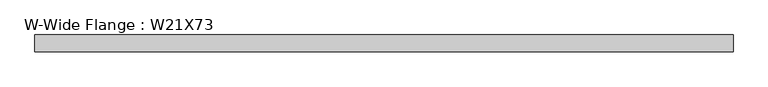
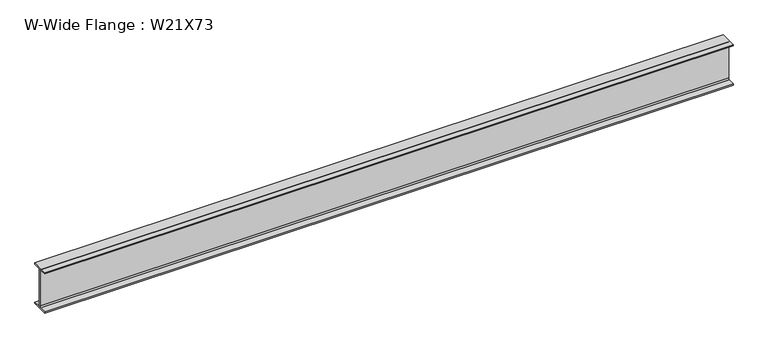
"""IFC4 building model written with IfcOpenShell, lengths in millimetres: beam geometry, W-Wide Flange : W21X73."""

import ifcopenshell
import ifcopenshell.guid

model = None  # the IFC model being written
_history = None  # IfcOwnerHistory: only IFC2X3 demands one
_inside = {}  # id of a spatial element -> (the spatial element, [elements in it])
_under = {}  # id of a project, library or spatial element -> (it, [spatial elements below it])
_declared = {}  # id of a project -> (the project, [libraries it declares])
_typed = {}  # id of a type object -> (the type object, [elements of that type])
_made_of = {}  # id of a material, layer set ... -> (it, [elements and type objects made of it])


def new_model(schema):
    """Start an empty IFC model of exactly this schema.

    Asked for "IFC4X3", IfcOpenShell would pick the latest addendum, in which some entities
    have other attributes; the version numbers below select the first issue.
    IFC2X3 requires an IfcOwnerHistory on every rooted entity: one is made here for all.
    """
    global model, _history
    if schema == "IFC4X3":
        model = ifcopenshell.file(schema_version=(4, 3, 0, 0))
    else:
        model = ifcopenshell.file(schema=schema)
    _inside.clear()
    _under.clear()
    _declared.clear()
    _typed.clear()
    _made_of.clear()
    _history = None
    if model.schema == "IFC2X3":
        org = make("IfcOrganization", Name="unknown")
        user = make(
            "IfcPersonAndOrganization",
            ThePerson=make("IfcPerson", FamilyName="unknown"),
            TheOrganization=org,
        )
        app = make(
            "IfcApplication",
            ApplicationDeveloper=org,
            Version="unknown",
            ApplicationFullName="unknown",
            ApplicationIdentifier="unknown",
        )
        _history = make(
            "IfcOwnerHistory",
            OwningUser=user,
            OwningApplication=app,
            ChangeAction="ADDED",
            CreationDate=0,
        )
    return model


def make(cls, **values):
    """One entity of the class cls with the attributes given. An attribute that is None is left unset."""
    return model.create_entity(
        cls, **{name: value for name, value in values.items() if value is not None}
    )


def rooted(cls, **values):
    """An entity with a GlobalId (a new one), such as an element, a storey or a relation."""
    return make(cls, GlobalId=ifcopenshell.guid.new(), OwnerHistory=_history, **values)


def si_unit(unit_type, name, prefix=None):
    """IfcSIUnit, for example si_unit("LENGTHUNIT", "METRE", prefix="MILLI")."""
    return make("IfcSIUnit", UnitType=unit_type, Prefix=prefix, Name=name)


def assignment(units):
    """IfcUnitAssignment: the units of a project."""
    return None if units is None else make("IfcUnitAssignment", Units=units)


def point(xyz):
    """IfcCartesianPoint."""
    return None if xyz is None else make("IfcCartesianPoint", Coordinates=xyz)


def direction(xyz):
    """IfcDirection."""
    return None if xyz is None else make("IfcDirection", DirectionRatios=xyz)


def frame(location, z_axis=None, x_axis=None):
    """IfcAxis2Placement3D, a coordinate frame: its origin and axes. An axis left out is left unset."""
    return make(
        "IfcAxis2Placement3D",
        Location=point(location),
        Axis=direction(z_axis),
        RefDirection=direction(x_axis),
    )


def frame_2d(location, x_axis=None):
    """IfcAxis2Placement2D, a coordinate frame in the plane: its origin and x axis."""
    return make(
        "IfcAxis2Placement2D", Location=point(location), RefDirection=direction(x_axis)
    )


def origin():
    """The frame at (0, 0, 0) with its axes left unset."""
    return frame((0.0, 0.0, 0.0))


def place(relative_to, where):
    """IfcLocalPlacement: puts the frame where relative to a parent placement (None: the world)."""
    return make(
        "IfcLocalPlacement", PlacementRelTo=relative_to, RelativePlacement=where
    )


def context(
    kind, dimensions, precision=None, world=None, true_north=None, identifier=None
):
    """IfcGeometricRepresentationContext, for example the 3D "Model" context."""
    return make(
        "IfcGeometricRepresentationContext",
        ContextIdentifier=identifier,
        ContextType=kind,
        CoordinateSpaceDimension=dimensions,
        Precision=precision,
        WorldCoordinateSystem=world,
        TrueNorth=true_north,
    )


def project(units=None, contexts=None):
    """IfcProject with its units and contexts."""
    return rooted(
        "IfcProject",
        Name="project",
        RepresentationContexts=contexts,
        UnitsInContext=assignment(units),
    )


def spatial(cls, under=None, at=None, **own):
    """A site, building, storey or space (cls), placed at a placement, below another one or the project."""
    s = rooted(cls, ObjectPlacement=at, **own)
    if under is not None:
        _under.setdefault(under.id(), (under, []))[1].append(s)
    return s


def polyline(points):
    """IfcPolyline through the points."""
    return make("IfcPolyline", Points=[point(p) for p in points])


def circle_curve(where, radius):
    """IfcCircle in the frame where."""
    return make("IfcCircle", Position=where, Radius=radius)


def trimmed(basis, trim1, trim2, sense, master):
    """IfcTrimmedCurve: the piece of a basis curve between two trims."""
    return make(
        "IfcTrimmedCurve",
        BasisCurve=basis,
        Trim1=trim1,
        Trim2=trim2,
        SenseAgreement=sense,
        MasterRepresentation=master,
    )


def segment(curve, same_sense, transition):
    """IfcCompositeCurveSegment."""
    return make(
        "IfcCompositeCurveSegment",
        Transition=transition,
        SameSense=same_sense,
        ParentCurve=curve,
    )


def composite_curve(segments, self_intersect=None):
    """IfcCompositeCurve: segments joined end to end."""
    return make("IfcCompositeCurve", Segments=segments, SelfIntersect=self_intersect)


def outline(outer, holes=None, kind="AREA"):
    """IfcArbitraryClosedProfileDef: a profile drawn as a closed curve; with holes, ...WithVoids."""
    if holes is None:
        return make("IfcArbitraryClosedProfileDef", ProfileType=kind, OuterCurve=outer)
    return make(
        "IfcArbitraryProfileDefWithVoids",
        ProfileType=kind,
        OuterCurve=outer,
        InnerCurves=holes,
    )


def extrude(swept, where, along, depth):
    """IfcExtrudedAreaSolid: the profile swept, set in the frame where, extruded along a direction by depth."""
    return make(
        "IfcExtrudedAreaSolid",
        SweptArea=swept,
        Position=where,
        ExtrudedDirection=direction(along),
        Depth=depth,
    )


def shape(context_of_items, identifier, shape_type, items):
    """IfcShapeRepresentation: the items that make up one representation, for example the "Body"."""
    return make(
        "IfcShapeRepresentation",
        ContextOfItems=context_of_items,
        RepresentationIdentifier=identifier,
        RepresentationType=shape_type,
        Items=items,
    )


def source(mapping_origin, context_of_items, identifier, shape_type, items):
    """IfcRepresentationMap: a shape defined once, which mapped items show again and again."""
    return make(
        "IfcRepresentationMap",
        MappingOrigin=mapping_origin,
        MappedRepresentation=shape(context_of_items, identifier, shape_type, items),
    )


def transform(
    local_origin,
    x_axis=None,
    y_axis=None,
    z_axis=None,
    scale=None,
    scale2=None,
    scale3=None,
    uniform=True,
):
    """IfcCartesianTransformationOperator3D, or its non-uniform kind. x_axis, y_axis, z_axis: its Axis1, 2, 3."""
    if uniform:
        return make(
            "IfcCartesianTransformationOperator3D",
            Axis1=direction(x_axis),
            Axis2=direction(y_axis),
            LocalOrigin=point(local_origin),
            Scale=scale,
            Axis3=direction(z_axis),
        )
    return make(
        "IfcCartesianTransformationOperator3DnonUniform",
        Axis1=direction(x_axis),
        Axis2=direction(y_axis),
        LocalOrigin=point(local_origin),
        Scale=scale,
        Axis3=direction(z_axis),
        Scale2=scale2,
        Scale3=scale3,
    )


def mapped(mapping_source, mapping_target):
    """IfcMappedItem: shows the shape of a source again, moved by a transform."""
    return make(
        "IfcMappedItem", MappingSource=mapping_source, MappingTarget=mapping_target
    )


def made_of(thing, what):
    """Note that an element or type object is made of a material, layer set ...; save() writes the relation."""
    if what is not None:
        _made_of.setdefault(what.id(), (what, []))[1].append(thing)
    return thing


def element(
    cls,
    number,
    at=None,
    inside=None,
    cuts=None,
    type_object=None,
    material=None,
    context=None,
    identifier="Body",
    shape_type=None,
    held_by="IfcProductDefinitionShape",
    body=None,
    shapes=None,
    **own,
):
    """One element of the class cls, such as IfcWall. Its Tag is "e" and its number.

    at: its placement. inside: the storey or other place that contains it. cuts: it is an
    opening in that element (IfcRelVoidsElement). A single representation is given by context,
    identifier, shape_type and body (its items); several are given by shapes. held_by: the class
    of the entity that holds the representations. save() writes the other relations.
    """
    e = rooted(cls, Tag="e%d" % number, ObjectPlacement=at, **own)
    if body is not None:
        shapes = [shape(context, identifier, shape_type, body)]
    if shapes is not None:
        e.Representation = make(held_by, Representations=shapes)
    if inside is not None:
        _inside.setdefault(inside.id(), (inside, []))[1].append(e)
    if cuts is not None:
        rooted(
            "IfcRelVoidsElement", RelatingBuildingElement=cuts, RelatedOpeningElement=e
        )
    if type_object is not None:
        _typed.setdefault(type_object.id(), (type_object, []))[1].append(e)
    return made_of(e, material)


def aggregate(whole, parts):
    """IfcRelAggregates: a whole, such as a stair, and the parts it consists of."""
    return rooted("IfcRelAggregates", RelatingObject=whole, RelatedObjects=parts)


def save(model, path):
    """Write the relations noted so far, then the file.

    IfcRelAggregates (storeys below a building ...), IfcRelContainedInSpatialStructure (elements
    in a storey), IfcRelDefinesByType, IfcRelAssociatesMaterial and IfcRelDeclares: one each for
    every whole, place, type object, material and project.
    """
    for whole, parts in _under.values():
        aggregate(whole, parts)
    for where, things in _inside.values():
        rooted(
            "IfcRelContainedInSpatialStructure",
            RelatedElements=things,
            RelatingStructure=where,
        )
    for kind, things in _typed.values():
        rooted("IfcRelDefinesByType", RelatedObjects=things, RelatingType=kind)
    for what, things in _made_of.values():
        rooted("IfcRelAssociatesMaterial", RelatedObjects=things, RelatingMaterial=what)
    for by, libraries in _declared.values():
        rooted("IfcRelDeclares", RelatingContext=by, RelatedDefinitions=libraries)
    model.write(path)


def w_wide_flange_w21x73_23efea6e(model_context):
    return source(origin(), model_context, "Body", "SweptSolid", [
        extrude(outline(composite_curve([segment(polyline([(105.41, -250.444), (105.41, -269.24), (-105.41, -269.24), (-105.41, -250.444), (-23.495, -250.444)]), True, "CONTINUOUS"), segment(trimmed(circle_curve(frame_2d((-23.495, -232.7275)), 17.7165), [point((-23.495, -250.444))], [point((-5.7785, -232.7275))], True, "CARTESIAN"), True, "CONTINUOUS"), segment(polyline([(-5.7785, -232.7275), (-5.7785, 232.7275)]), True, "CONTINUOUS"), segment(trimmed(circle_curve(frame_2d((-23.495, 232.7275)), 17.7165), [point((-5.7785, 232.7275))], [point((-23.495, 250.444))], True, "CARTESIAN"), True, "CONTINUOUS"), segment(polyline([(-23.495, 250.444), (-105.41, 250.444), (-105.41, 269.24), (105.41, 269.24), (105.41, 250.444), (23.495, 250.444)]), True, "CONTINUOUS"), segment(trimmed(circle_curve(frame_2d((23.495, 232.7275)), 17.7165), [point((23.495, 250.444))], [point((5.7785, 232.7275))], True, "CARTESIAN"), True, "CONTINUOUS"), segment(polyline([(5.7785, 232.7275), (5.7785, -232.7275)]), True, "CONTINUOUS"), segment(trimmed(circle_curve(frame_2d((23.495, -232.7275)), 17.7165), [point((5.7785, -232.7275))], [point((23.495, -250.444))], True, "CARTESIAN"), True, "CONTINUOUS"), segment(polyline([(23.495, -250.444), (105.41, -250.444)]), True, "CONTINUOUS")], self_intersect=False)), frame((-4324.35, 0.0, 0.0), z_axis=(1.0, 0.0, 0.0), x_axis=(0.0, 1.0, 0.0)), (0.0, 0.0, 1.0), 8648.7),
    ])


if __name__ == "__main__":
    model = new_model("IFC4")
    model_context = context("Model", 3, world=origin())
    ifc_project = project(units=[si_unit("LENGTHUNIT", "METRE", prefix="MILLI")], contexts=[model_context])
    site = spatial("IfcSite", under=ifc_project)
    building = spatial("IfcBuilding", under=site)
    placement = place(None, origin())
    w_wide_flange_w21x73_shape = w_wide_flange_w21x73_23efea6e(model_context)
    element("IfcBeam", 1, ObjectType="W-Wide Flange : W21X73", at=placement, inside=building, context=model_context, shape_type="MappedRepresentation", body=[
        mapped(w_wide_flange_w21x73_shape, transform((0.0, 0.0, 0.0), x_axis=(1.0, 0.0, 0.0), y_axis=(0.0, 1.0, 0.0), z_axis=(0.0, 0.0, 1.0))),
    ])
    save(model, "model.ifc")

# Revit data of these elements
# Type "W-Wide Flange : W21X73"
#   Assembly Code = "B10"
#   W = 73
#   Start Extension Calculation [instance default] = 10' - 0"
#   Start Extension [instance default] = -0' - 0 1/2"
#   End Extension Calculation [instance default] = 10' - 0"
#   End Extension [instance default] = -0' - 0 1/2"
#   Length [instance default] = 5' - 0"
#   bf = 0' - 8.3"
#   d = 1' - 9.2"
#   k = 0' - 1 7/16"
#   k2 = 0' - 0.6975"
#   tf = 0' - 0.74"
#   tw = 0' - 0.455"
#   A = 0.149306 SF
#   Beam Material [instance default] = Metal - Steel - ASTM A992
# Element 1 (IfcBeam, "W-Wide Flange : W21X73")
#   Materials on its faces: "Metal - Steel - ASTM A992"
# Materials
#   "Metal - Steel - ASTM A992": class "Metal", colour RGB 128 0 0, transparency 0
